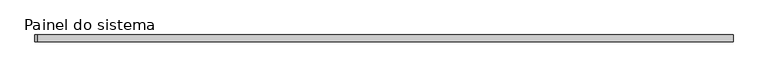
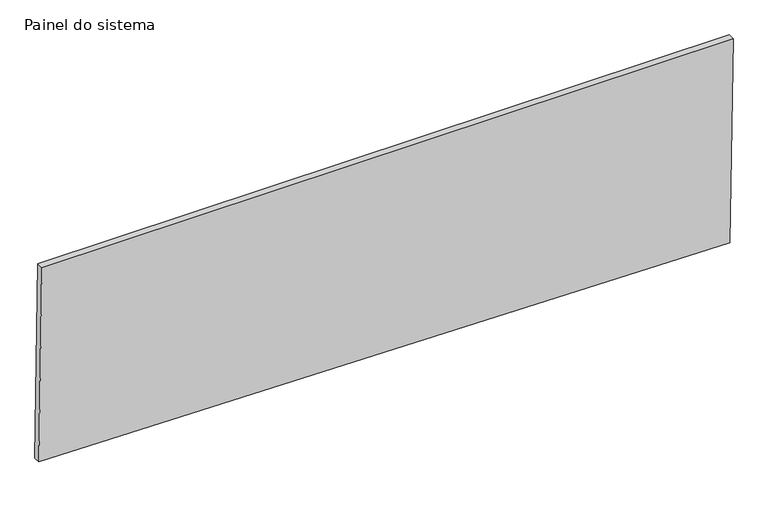
"""IFC4 building model written with IfcOpenShell, lengths in millimetres: plate geometry, Painel do sistema : Envidraçado."""

from ifc_helpers import new_model, si_unit, frame, origin, place, context, project, spatial, polyline, outline, extrude, source, transform, mapped, element, save


def painel_do_sistema_13cd06c8(model_context):
    return source(origin(), model_context, "Body", "SweptSolid", [
        extrude(outline(polyline([(37.9368749, -1267.0645365), (0.0, 1255.2791262), (783.5873474, 1267.0645365), (783.5873474, -1255.8497092), (37.9368749, -1267.0645365)])), frame((0.0, 24.5, 0.0), z_axis=(0.0, 1.0, 0.0), x_axis=(0.0, 0.0, 1.0)), (0.0, 0.0, 1.0), 25.0),
    ])


if __name__ == "__main__":
    model = new_model("IFC4")
    model_context = context("Model", 3, world=origin())
    ifc_project = project(units=[si_unit("LENGTHUNIT", "METRE", prefix="MILLI")], contexts=[model_context])
    site = spatial("IfcSite", under=ifc_project)
    building = spatial("IfcBuilding", under=site)
    placement = place(None, origin())
    painel_do_sistema_shape = painel_do_sistema_13cd06c8(model_context)
    element("IfcPlate", 1, ObjectType="Painel do sistema : Envidraçado", at=placement, inside=building, context=model_context, shape_type="MappedRepresentation", body=[
        mapped(painel_do_sistema_shape, transform((0.0, 0.0, 0.0), x_axis=(1.0, 0.0, 0.0), y_axis=(0.0, 1.0, 0.0), z_axis=(0.0, 0.0, 1.0))),
    ])
    save(model, "model.ifc")

# Revit data of these elements
# Type "Painel do sistema : Envidraçado"
#   Construction Type Id = "GSP4R"
#   Analytic Construction = "Vidraça única Pilkington 1/8 pol"
#   Visual Light Transmittance = 0.9
#   Solar Heat Gain Coefficient = 0.86
#   Heat Transfer Coefficient (U) = 6.7069 W/(m²·K)
# Element 1 (IfcPlate, "Painel do sistema : Envidraçado")
#   Materials on its faces: "Vidro"
# Materials
#   "Vidro": class "Vidro", colour RGB 0 128 192, transparency 0.9, Description = "Vidro de sílica", Cost = 0
